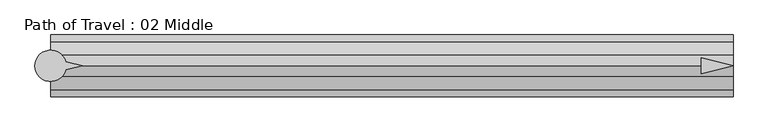
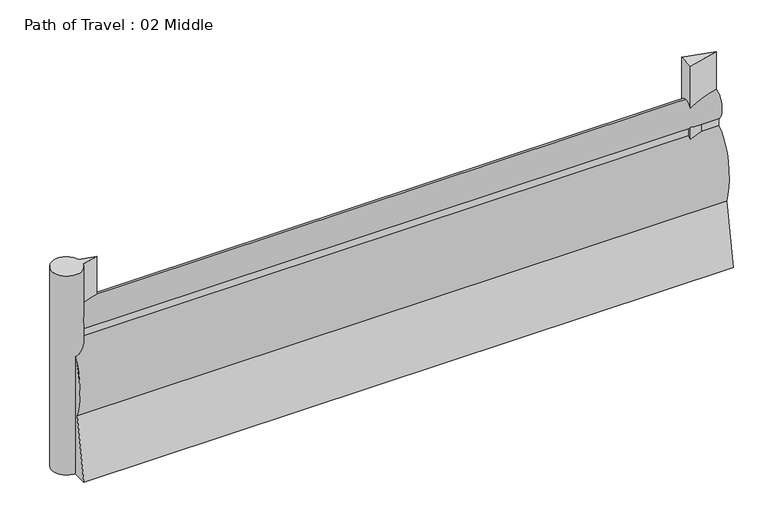
"""IFC4 building model written with IfcOpenShell, lengths in millimetres: proxy geometry, Path of Travel : 02 Middle."""

from ifc_helpers import new_model, si_unit, point, frame, frame_2d, origin, origin_with_axes, place, context, project, spatial, polyline, circle_curve, ellipse_curve, trimmed, segment, composite_curve, outline, extrude, source, transform, mapped, element, save
from ifc_brep_helpers import plane_surface, extruded_surface, advanced_brep


def path_of_travel_02_middle_1f19553c(model_context):
    return source(origin(), model_context, "Body", "SolidModel", [
        advanced_brep(
        [(227.5554837, 0.0, 1727.2), (227.5554837, 42.9018657, 1436.6534209), (227.5554837, 42.9018657, 1363.4763406), (227.5554837, 184.1186263, 643.4144547), (227.5554837, 297.5699544, 0.0), (227.5554837, 145.6574193, 0.0), (227.5554837, 0.0, 584.2), (227.5554837, -145.6574193, 0.0), (227.5554837, -297.5699544, 0.0), (227.5554837, -184.1186263, 643.4144547), (227.5554837, -42.9018657, 1363.4763406), (227.5554837, -42.9018657, 1436.6534209), (6800.4193593, 0.0, 1727.2), (6800.4193593, -42.9018657, 1436.6534209), (6800.4193593, -42.9018657, 1363.4763406), (6800.4193593, -184.1186263, 643.4144547), (6800.4193593, -297.5699544, 0.0), (6800.4193593, -145.6574193, 0.0), (6800.4193593, 0.0, 584.2), (6800.4193593, 145.6574193, 0.0), (6800.4193593, 297.5699544, 0.0), (6800.4193593, 184.1186263, 643.4144547), (6800.4193593, 42.9018657, 1363.4763406), (6800.4193593, 42.9018657, 1436.6534209)],
        [
            (0, 1, ellipse_curve(frame((227.5554837, 0.0, 1574.8), z_axis=(-1.0, 0.0, 0.0), x_axis=(0.0, 0.0, 1.0)), 152.4, 101.6)),
            (1, 2),
            (2, 3, ellipse_curve(frame((227.5554837, 0.0, 914.4), z_axis=(-1.0, 0.0, 0.0), x_axis=(0.0, 0.0, -1.0)), 457.2, 228.6)),
            (3, 4),
            (4, 5),
            (5, 6),
            (6, 7),
            (7, 8),
            (8, 9),
            (9, 10, ellipse_curve(frame((227.5554837, 0.0, 914.4), z_axis=(-1.0, 0.0, 0.0), x_axis=(0.0, 0.0, -1.0)), 457.2, 228.6)),
            (10, 11),
            (11, 0, ellipse_curve(frame((227.5554837, 0.0, 1574.8), z_axis=(-1.0, 0.0, 0.0), x_axis=(0.0, 0.0, 1.0)), 152.4, 101.6)),
            (12, 13, ellipse_curve(frame((6800.4193593, 0.0, 1574.8), z_axis=(1.0, 0.0, 0.0), x_axis=(0.0, 0.0, 1.0)), 152.4, 101.6)),
            (13, 14),
            (14, 15, ellipse_curve(frame((6800.4193593, 0.0, 914.4), z_axis=(1.0, 0.0, 0.0), x_axis=(0.0, 0.0, -1.0)), 457.2, 228.6)),
            (15, 16),
            (16, 17),
            (17, 18),
            (18, 19),
            (19, 20),
            (20, 21),
            (21, 22, ellipse_curve(frame((6800.4193593, 0.0, 914.4), z_axis=(1.0, 0.0, 0.0), x_axis=(0.0, 0.0, -1.0)), 457.2, 228.6)),
            (22, 23),
            (23, 12, ellipse_curve(frame((6800.4193593, 0.0, 1574.8), z_axis=(1.0, 0.0, 0.0), x_axis=(0.0, 0.0, 1.0)), 152.4, 101.6)),
            (0, 12),
            (23, 1),
            (22, 2),
            (21, 3),
            (20, 4),
            (19, 5),
            (18, 6),
            (17, 7),
            (16, 8),
            (15, 9),
            (14, 10),
            (13, 11),
        ],
        [
            plane_surface(frame((227.5554837, 0.0, 0.0), z_axis=(-1.0, 0.0, 0.0), x_axis=(0.0, 0.0, 1.0))),
            plane_surface(frame((6800.4193593, 0.0, 0.0), z_axis=(1.0, 0.0, 0.0), x_axis=(0.0, 0.0, 1.0))),
            extruded_surface(trimmed(ellipse_curve(frame((6800.4193593, 0.0, 1574.8), z_axis=(-1.0, 0.0, 0.0), x_axis=(0.0, 0.0, 1.0)), 152.4, 101.6), [point((6800.4193593, 0.0, 1727.2))], [point((6800.4193593, 42.9018657, 1436.6534209))], True, "CARTESIAN"), (-6572.8638756, 0.0, 0.0), 6572.8638756),
            plane_surface(frame((227.5554837, 42.9018657, 1436.6534209), z_axis=(0.0, 1.0, 0.0), x_axis=(1.0, 0.0, 0.0))),
            extruded_surface(trimmed(ellipse_curve(frame((6800.4193593, 0.0, 914.4), z_axis=(-1.0, 0.0, 0.0), x_axis=(0.0, 0.0, -1.0)), 457.2, 228.6), [point((6800.4193593, 42.9018657, 1363.4763406))], [point((6800.4193593, 184.1186263, 643.4144547))], True, "CARTESIAN"), (-6572.8638756, 0.0, 0.0), 6572.8638756),
            plane_surface(frame((227.5554837, 184.1186263, 643.4144547), z_axis=(0.0, 0.9848077530122078, 0.1736481776669322), x_axis=(1.0, 0.0, 0.0))),
            plane_surface(frame((227.5554837, 297.5699544, 0.0), z_axis=(0.0, 0.0, -1.0), x_axis=(1.0, 0.0, 0.0))),
            plane_surface(frame((227.5554837, 145.6574193, 0.0), z_axis=(0.0, -0.9702957262760199, -0.2419218955995739), x_axis=(1.0, 0.0, 0.0))),
            plane_surface(frame((227.5554837, 0.0, 584.2), z_axis=(0.0, 0.9702957262759961, -0.24192189559966923), x_axis=(1.0, 0.0, 0.0))),
            plane_surface(frame((227.5554837, -145.6574193, 0.0), z_axis=(0.0, 0.0, -1.0), x_axis=(1.0, 0.0, 0.0))),
            plane_surface(frame((227.5554837, -297.5699544, 0.0), z_axis=(0.0, -0.984807753012208, 0.17364817766693066), x_axis=(1.0, 0.0, 0.0))),
            extruded_surface(trimmed(ellipse_curve(frame((6800.4193593, 0.0, 914.4), z_axis=(-1.0, 0.0, 0.0), x_axis=(0.0, 0.0, -1.0)), 457.2, 228.6), [point((6800.4193593, -184.1186263, 643.4144547))], [point((6800.4193593, -42.9018657, 1363.4763406))], True, "CARTESIAN"), (-6572.8638756, 0.0, 0.0), 6572.8638756),
            plane_surface(frame((227.5554837, -42.9018657, 1363.4763406), z_axis=(0.0, -1.0, 0.0), x_axis=(1.0, 0.0, 0.0))),
            extruded_surface(trimmed(ellipse_curve(frame((6800.4193593, 0.0, 1574.8), z_axis=(-1.0, 0.0, 0.0), x_axis=(0.0, 0.0, 1.0)), 152.4, 101.6), [point((6800.4193593, -42.9018657, 1436.6534209))], [point((6800.4193593, 0.0, 1727.2))], True, "CARTESIAN"), (-6572.8638756, 0.0, 0.0), 6572.8638756),
        ],
        [
            (0, [[1, 2, 3, 4, 5, 6, 7, 8, 9, 10, 11, 12]]),
            (1, [[13, 14, 15, 16, 17, 18, 19, 20, 21, 22, 23, 24]]),
            (2, [[-1, 25, -24, 26]]),
            (3, [[-2, -26, -23, 27]]),
            (4, [[-3, -27, -22, 28]]),
            (5, [[-4, -28, -21, 29]]),
            (6, [[-5, -29, -20, 30]]),
            (7, [[-6, -30, -19, 31]]),
            (8, [[-7, -31, -18, 32]]),
            (9, [[-8, -32, -17, 33]]),
            (10, [[-9, -33, -16, 34]]),
            (11, [[-10, -34, -15, 35]]),
            (12, [[-11, -35, -14, 36]]),
            (13, [[-12, -36, -13, -25]]),
        ],
    ),
        extrude(outline(polyline([(6494.4142127, 76.2006338), (6800.4193593, 0.0), (6494.4142127, -76.2006338), (6494.4142127, 76.2006338)])), origin_with_axes(), (0.0, 0.0, 1.0), 2129.5973753),
        extrude(outline(composite_curve([segment(polyline([(372.7837828, 39.4440225), (531.182385, 0.0), (372.7837828, -39.4440225)]), True, "CONTINUOUS"), segment(trimmed(circle_curve(frame_2d((227.2200886, 0.0)), 150.8131956), [point((372.7837828, -39.4440225))], [point((372.7837828, 39.4440225))], False, "CARTESIAN"), True, "CONTINUOUS")], self_intersect=False)), origin_with_axes(), (0.0, 0.0, 1.0), 2129.5973753),
    ])


if __name__ == "__main__":
    model = new_model("IFC4")
    model_context = context("Model", 3, world=origin())
    ifc_project = project(units=[si_unit("LENGTHUNIT", "METRE", prefix="MILLI")], contexts=[model_context])
    site = spatial("IfcSite", under=ifc_project)
    building = spatial("IfcBuilding", under=site)
    placement = place(None, origin())
    path_of_travel_02_middle_shape = path_of_travel_02_middle_1f19553c(model_context)
    element("IfcBuildingElementProxy", 1, Name="Path of Travel : 02 Middle", ObjectType="Path of Travel : 02 Middle", at=placement, inside=building, context=model_context, shape_type="MappedRepresentation", body=[
        mapped(path_of_travel_02_middle_shape, transform((0.0, 0.0, 0.0), x_axis=(1.0, 0.0, 0.0), y_axis=(0.0, 1.0, 0.0), z_axis=(0.0, 0.0, 1.0))),
    ])
    save(model, "model.ifc")

# Revit data of these elements
# Type "Path of Travel : 02 Middle"
#   Path of Egress [instance default] = 4' - 0"
#   built-in parameter 1001306 [instance default] = 4 (stored number, unit not read)
#   Dot at Start = no
#   Arrow in Middle = yes
#   Arrow at End = no
#   Egress Path = none
# Element 1 (IfcBuildingElementProxy, "Path of Travel : 02 Middle")
#   Path of Egress = 21' - 6.77417"
#   built-in parameter 1001306 = 21.5645 (stored number, unit not read)
#   Materials on its faces: "Egress Path Solid", "solid"
# Materials
#   "Egress Path Solid": class "Unassigned", colour RGB 255 128 64, transparency 0.75, Comments = "Rendering appearance not upgraded "
#   "solid": class "Generic", colour RGB 120 120 120, transparency 0, Cost = 0
